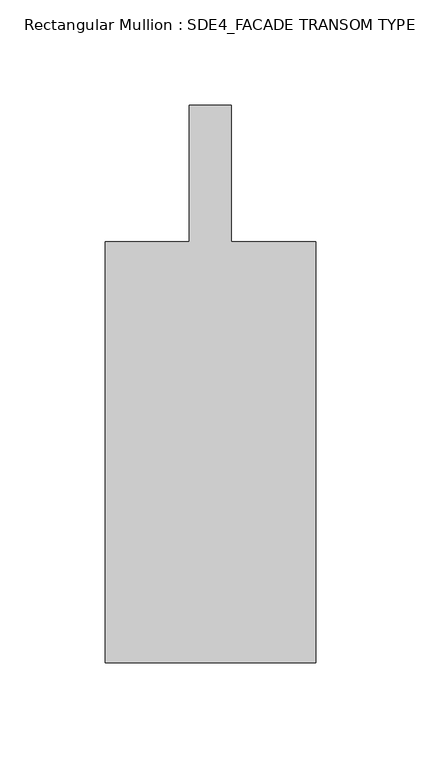
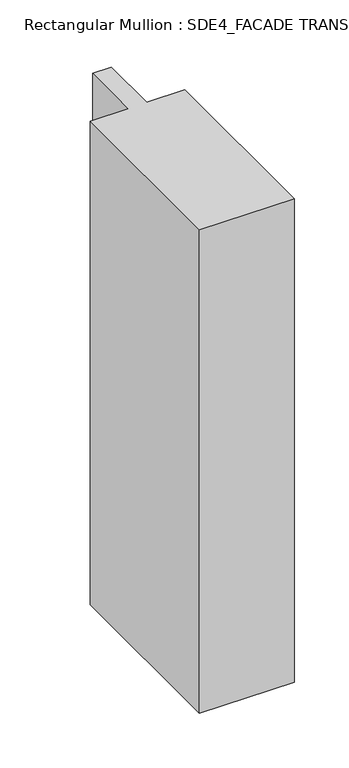
"""IFC4 building model written with IfcOpenShell, lengths in millimetres: member geometry, Rectangular Mullion : SDE4_FACADE TRANSOM TYPE 2."""

from ifc_helpers import new_model, si_unit, frame, origin, place, context, project, spatial, polyline, outline, extrude, source, transform, mapped, element, save


def rectangular_mullion_sde4_facade_transom_type_2_e057eab3(model_context):
    return source(origin(), model_context, "Body", "SweptSolid", [
        extrude(outline(polyline([(50.0, -132.5), (-50.0, -132.5), (-50.0, 67.5), (-10.0, 67.5), (-10.0, 132.5), (10.0, 132.5), (10.0, 67.5), (50.0, 67.5), (50.0, -132.5)])), frame((0.0, 0.0, -540.06364), z_axis=(0.0, 0.0, 1.0), x_axis=(1.0, 0.0, 0.0)), (0.0, 0.0, 1.0), 540.06364),
    ])


if __name__ == "__main__":
    model = new_model("IFC4")
    model_context = context("Model", 3, world=origin())
    ifc_project = project(units=[si_unit("LENGTHUNIT", "METRE", prefix="MILLI")], contexts=[model_context])
    site = spatial("IfcSite", under=ifc_project)
    building = spatial("IfcBuilding", under=site)
    placement = place(None, origin())
    rectangular_mullion_sde4_facade_transom_type_2_shape = rectangular_mullion_sde4_facade_transom_type_2_e057eab3(model_context)
    element("IfcMember", 1, ObjectType="Rectangular Mullion : SDE4_FACADE TRANSOM TYPE 2", at=placement, inside=building, context=model_context, shape_type="MappedRepresentation", body=[
        mapped(rectangular_mullion_sde4_facade_transom_type_2_shape, transform((0.0, 0.0, 0.0), x_axis=(1.0, 0.0, 0.0), y_axis=(0.0, 1.0, 0.0), z_axis=(0.0, 0.0, 1.0))),
    ])
    save(model, "model.ifc")

# Revit data of these elements
# Type "Rectangular Mullion : SDE4_FACADE TRANSOM TYPE 2"
#   built-in parameter 1007322 = 0.869423 (stored number, unit not read)
#   built-in parameter 1007321 = 0.164042 (stored number, unit not read)
#   built-in parameter 1007320 = 0.164042 (stored number, unit not read)
